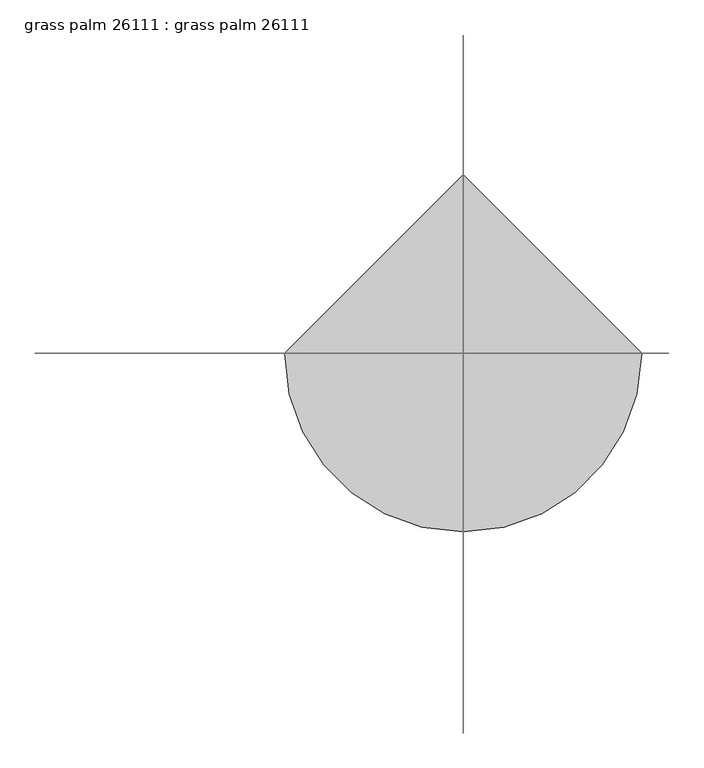
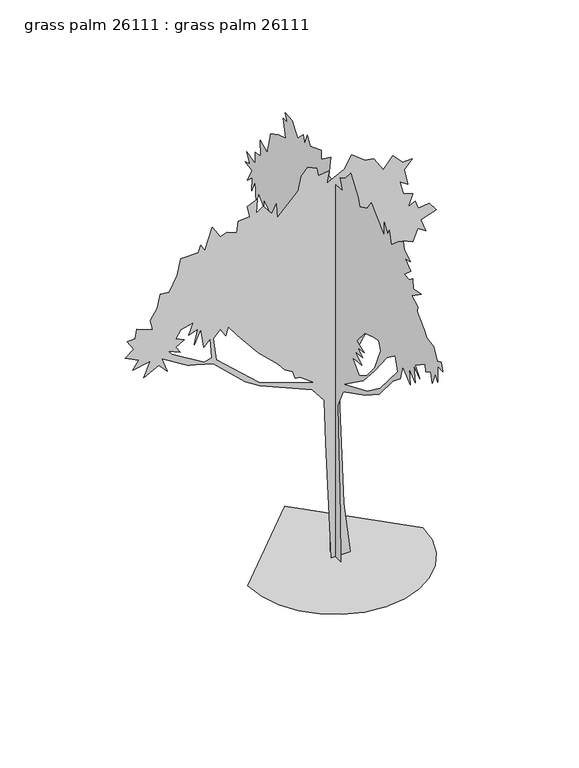
"""IFC4 building model written with IfcOpenShell, lengths in millimetres: proxy geometry, grass palm 26111 : grass palm 26111."""

from ifc_helpers import new_model, si_unit, origin, place, context, project, spatial, triangles, source, transform, mapped, element, save


def grass_palm_26111_grass_palm_26111_ffc4a38a(model_context):
    return source(origin(), model_context, "Body", "Tessellation", [
        triangles([(197.8251161, -0.0004657, 0.0001367), (109.1148514, -0.0002635, 694.5605118), (43.5490633, 0.0002048, 2380.5060047), (409.1686295, 0.0003079, 2962.5546341), (570.4154732, 0.000405, 3409.2137077), (607.6747178, 0.0004576, 3623.4372597), (719.4525244, 0.0004509, 3660.6992294), (654.2481468, 0.0004936, 3781.8063721), (747.397621, 0.0005252, 3949.4717194), (775.3401741, 0.0005007, 3874.9480705), (877.80376, 0.0005308, 4042.6134178), (1008.2098989, 0.0004934, 3977.4115837), (1073.4142765, 0.0005291, 4145.0772217), (1175.8753189, 0.0004934, 4070.5535728), (1110.6734848, 0.0005514, 4247.5407349), (1315.5981857, 0.0005381, 4312.742569), (1222.4487843, 0.0005851, 4433.8244225), (1082.7284609, 0.0006012, 4415.2060822), (1039.2334414, 0.0006388, 4529.6586891), (952.3222492, 0.0006386, 4480.4079163), (1008.2098989, 0.0006732, 4638.7514488), (886.9528381, 0.0007051, 4688.7640938), (840.544479, 0.0007593, 4862.3223953), (943.0055214, 0.0007261, 4797.0952721), (896.4321287, 0.0007914, 5011.3441132), (998.8957146, 0.0008063, 5123.1297318), (877.80376, 0.0008246, 5123.1297318), (747.397621, 0.0008797, 5253.5334), (626.3056664, 0.0008575, 5104.4861023), (503.8725509, 0.0009294, 5301.1072403), (384.1216845, 0.0009523, 5318.7352341), (216.4545022, 0.0010156, 5458.4604263), (113.9921609, 0.0009855, 5290.795079), (-109.5623986, 0.0009889, 5179.0094604), (-81.6183375, 0.0010277, 5337.3532837), (-221.3396873, 0.0010437, 5318.7352341), (-239.9693097, 0.0010769, 5430.5202713), (-361.0610281, 0.0011104, 5486.4005814), (-444.8937381, 0.0010978, 5393.2585922), (-482.1529827, 0.0010527, 5206.9496155), (-752.2819885, 0.0010175, 4927.5242294), (-770.9103573, 0.0010735, 5123.1297318), (-826.8005505, 0.0010516, 5011.3441132), (-938.5783207, 0.0011065, 5151.0698868), (-1031.7252514, 0.0011028, 5085.8680527), (-1013.0943392, 0.0011506, 5272.1514496), (-1143.5030216, 0.0011551, 5216.2711395), (-1115.557925, 0.0011104, 5067.2244232), (-1264.5950489, 0.0011304, 5057.9278976), (-1283.2232723, 0.0010926, 4908.8806), (-1404.3152996, 0.0011236, 4955.4643845), (-1497.4622303, 0.0011301, 4927.5242294), (-1599.9257435, 0.0011911, 5095.1895767), (-1702.389402, 0.0011281, 4806.4170868), (-1748.9628674, 0.0011604, 4899.5590759), (-1786.2220757, 0.0011407, 4806.4170868), (-2009.7751453, 0.0011745, 4806.4170868), (-2056.3486107, 0.0011233, 4592.1932442), (-2158.8122692, 0.0010856, 4396.5624527), (-2279.9041512, 0.0011064, 4405.8842674), (-2317.1635048, 0.0010639, 4228.8971054), (-2410.3102901, 0.00104, 4089.1972023), (-2377.0008408, 0.0009991, 3957.4473953), (-2587.2949814, 0.0010515, 4033.2916031), (-2605.9133217, 0.0010214, 3912.2100403), (-2708.3768349, 0.0010343, 3902.8882256), (-2624.5569511, 0.0009862, 3772.4845573), (-2736.3166992, 0.0009803, 3688.6390938), (-2559.355117, 0.0009282, 3595.4973953), (-2633.853186, 0.0009091, 3483.7117767), (-2410.3102901, 0.000888, 3530.2955612), (-2494.1431091, 0.0008475, 3334.6900589), (-2298.535136, 0.0008458, 3437.1535721), (-2186.7573658, 0.000796, 3316.0464294), (-2261.2733116, 0.0008604, 3511.6772209), (-1928.0074619, 0.0007539, 3305.1500015), (-1586.5374619, 0.000677, 3211.8556961), (-1169.4034029, 0.0005069, 2817.7745178), (-980.3029541, 0.0004448, 2694.5084953), (-299.9587802, 0.0002625, 2401.7378483), (-143.374379, 0.000185, 2203.9150394), (-126.1084725, 2.08e-05, 1609.6107628), (-53.6737587, -0.0004278, 0.0001367), (-1497.4622303, 0.0008957, 3651.4027039), (-1422.9462845, 0.000854, 3539.6173759), (-1395.0011879, 0.0008802, 3651.4027039), (-1273.9091606, 0.0008189, 3493.0335915), (-1002.0681953, 0.0003602, 3156.4073364), (-744.7432772, 0.0005791, 2905.2014488), (-659.9860233, 0.000538, 2801.1377426), (-556.6715083, 0.0005054, 2738.5520279), (-519.4122637, 0.0004719, 2636.0885147), (-454.2079225, 0.0004596, 2626.7667), (-267.9141337, 0.0003934, 2487.0438332), (-995.0831566, 0.0005747, 2749.8295372), (-1549.5677708, 0.0007954, 3253.765638), (-1590.6116318, 0.0008844, 3558.2354256), (-2019.0918732, 0.0008854, 3520.9737465), (-2074.9794502, 0.0009166, 3604.8192101), (-1963.20168, 0.0009175, 3670.0207535), (-2074.9794502, 0.0009495, 3725.9007729), (-2009.7751453, 0.0009676, 3828.3645767), (-1851.4239098, 0.0009538, 3865.6262558), (-1907.3141029, 0.0009217, 3716.604538), (-1791.7262455, 0.0009145, 3754.1964294), (-1838.0305412, 0.0008682, 3558.4641907), (-1748.9628674, 0.0009054, 3744.5444023), (-1711.7036591, 0.0008288, 3483.7117767), (-1627.8708401, 0.000839, 3567.5572403), (-1608.65835, 0.0007633, 3299.7651558), (-1708.7927902, 0.0007706, 3271.2916031), (-2130.8671726, 0.0009048, 3530.2955612), (-2177.4431087, 0.000927, 3586.1755806), (0.0001009, -125.9822357, 0.0001592), (6.27e-05, -114.0061317, 632.7801258), (3.21e-05, -52.0852428, 2115.3046051), (1.35e-05, -175.1038104, 2373.6836014), (-6.14e-05, -671.5328476, 2630.4243256), (-0.0001496, -990.5162842, 2836.0117767), (-0.0001562, -1298.9586491, 3200.2479744), (-0.0001816, -1467.3098557, 3334.6900589), (-0.00019, -1523.1974327, 3539.6173759), (-0.0002153, -1690.8629253, 3390.5700783), (-0.0002111, -1662.9202995, 3595.4973953), (-0.0002322, -1802.6406956, 3483.7373566), (-0.0002266, -1765.3814873, 3707.2827232), (-0.0002477, -1905.101738, 3604.8192101), (-0.0002322, -1802.6406956, 3725.9007729), (-0.000266, -2026.196236, 3874.9480705), (-0.0002688, -2044.8246048, 3781.8063721), (-0.0002843, -2147.2882633, 3837.6863914), (-0.0002899, -2184.5450008, 3707.2827232), (-0.0002997, -2249.7493057, 3874.9480705), (-0.0003096, -2314.9536106, 3800.4244217), (-0.0003096, -2314.9536106, 4023.9697884), (-0.0003265, -2426.7289101, 4014.6735535), (-0.0003208, -2389.4721725, 4126.4335922), (-0.0003068, -2296.3227711, 4079.8753876), (-0.0002955, -2221.8042091, 4238.2189201), (-0.0002716, -2063.4555897, 4266.1590752), (-0.0002632, -2007.5653965, 4340.6824333), (-0.0002792, -1849.2141609, 4489.729731), (-0.0002806, -1858.5282726, 4564.2280907), (-0.0002609, -1728.1221336, 4638.7514488), (-0.0002933, -1942.3609463, 4787.7987465), (-0.0002652, -1756.0672302, 4750.5370674), (-0.0002638, -1746.7531185, 4880.9404449), (-0.0002525, -1672.2345566, 4825.0607162), (-0.0002356, -1560.4567863, 4834.3569511), (-0.0002567, -1700.177037, 4955.4643845), (-0.0002384, -1579.0876259, 5057.9278976), (-0.0002553, -1690.8629253, 5085.8680527), (-0.0002342, -1551.1425293, 5169.6879364), (-0.0002314, -1532.5116898, 5262.854924), (-0.0002145, -1420.7339195, 5197.6530899), (-0.0001906, -1262.3826839, 5057.9278976), (-0.0001836, -1215.8092186, 5225.5932449), (-0.000178, -1178.5499376, 5151.0698868), (-0.0002067, -1104.0339191, 5272.1514496), (-0.0001667, -1104.0339191, 5085.8680527), (-0.0001811, -934.8191025, 5242.9666031), (-0.0001617, -805.9598167, 5355.9969131), (-0.0001497, -726.4933737, 5236.9472031), (-0.0001237, -554.4617231, 5151.0698868), (-0.0001181, -517.2024785, 5253.5334), (-9.28e-05, -349.5370585, 5486.4005814), (-7.45e-05, -228.4440684, 5346.6748077), (-5.62e-05, -107.3520956, 5281.4729736), (-6.46e-05, -163.2409807, 5132.4512558), (-4.21e-05, -14.2045188, 5123.1297318), (-1.82e-05, 144.1465339, 5151.0698868), (-2.38e-05, 106.8877798, 5430.5202713), (7.1e-06, 311.8129804, 5281.4729736), (7.1e-06, 311.8129804, 5402.5551178), (4.51e-05, 563.311074, 5309.4131287), (5.49e-05, 628.5154152, 5421.1987473), (6.48e-05, 693.7172493, 5262.854924), (6.9e-05, 721.6623459, 5365.3184372), (8.73e-05, 842.7543005, 5244.2112946), (9.71e-05, 907.9586054, 5309.4131287), (0.000107, 973.1604395, 5411.8766418), (9.09e-05, 1131.5116751, 5421.1987473), (0.0001238, 1084.9382097, 5318.7352341), (0.0001369, 1171.5319067, 5326.1010635), (0.0001281, 1112.8833063, 5085.8680527), (0.0001548, 1289.862838, 5020.6662186), (0.0001793, 1452.3822784, 4938.471817), (0.0001914, 1532.0468925, 4629.4296341), (0.0002153, 1690.3981281, 4703.9532829), (0.0002139, 1681.0838711, 4489.729731), (0.0002321, 1802.1758984, 4471.0861015), (0.0002321, 1802.1758984, 4312.742569), (0.0002617, 1997.7863422, 4359.3007736), (0.0002506, 1924.1873463, 4240.2763527), (0.0002671, 2033.8797787, 4204.1576271), (0.0002434, 1876.6944603, 4173.017086), (0.0002603, 1988.4722305, 3977.4115837), (0.000242, 1867.3802032, 4079.8753876), (0.0002448, 1886.008572, 3893.5664108), (0.0002321, 1802.1758984, 4070.5535728), (0.0002293, 1783.5475296, 3791.102607), (0.0002209, 1727.6573364, 3949.4717194), (0.000204, 1615.8795662, 3837.6863914), (0.000204, 1615.8795662, 3940.1499046), (0.0001974, 1307.620039, 3736.3911209), (0.0001385, 917.2727898, 3623.4372597), (0.0001194, 790.5928768, 3229.1531868), (0.0001184, 784.0523603, 3133.6235527), (0.0001019, 675.0888805, 3064.5609077), (0.0001273, 842.7543005, 2934.1575302), (0.0001104, 730.9765303, 2971.4192093), (0.0001532, 749.6048264, 2775.813707), (0.0001377, 647.143784, 2906.2173752), (0.0001349, 628.5154152, 2673.3501938), (0.0001307, 600.5703549, 2775.813707), (0.0001264, 572.6252584, 2673.3501938), (0.0001194, 526.0518293, 2841.0155411), (0.0001152, 498.1067327, 2682.6467194), (0.0001124, 479.478364, 2608.1483597), (0.0001067, 442.2191194, 2738.5520279), (9.69e-05, 377.0147781, 2654.7065643), (7.78e-05, 250.6550855, 2492.941729), (2.45e-05, 161.9890223, 2108.946999), (9.68e-05, 111.8545007, 1061.9156324), (0.0001375, 116.2017099, 0.0001159), (-9.51e-05, -630.0470804, 2801.0107155), (-0.0001338, -885.9978092, 3096.8699821), (-0.0001753, -1160.7521868, 3441.0905411), (-0.0002047, -1355.5320854, 3586.1755806), (-0.0002131, -1411.4196625, 3399.891893), (-0.0001538, -1018.750898, 2931.8969124), (-0.0001089, -721.0450871, 2712.8219124), (-2.89e-05, -191.1855686, 2487.0438332), (-6.83e-05, -451.9981009, 2980.7157349), (-8.93e-05, -591.7210041, 2990.0375496), (-6.83e-05, -451.9981009, 3092.5010628), (-9.36e-05, -619.6661007, 3111.1446922), (-7.67e-05, -507.7485861, 3183.8393829), (-9.92e-05, -656.9227655, 3204.2863907), (-7.39e-05, -489.2573819, 3269.4882248), (-0.0001003, -664.5148893, 3478.2763527), (-0.0001315, -871.1641943, 3548.9391907), (-0.0001484, -982.9419645, 3567.5572403), (-0.0001546, -1023.6937649, 3456.6608116), (-0.0001342, -889.0838854, 3136.1382248), (-0.0001091, -722.497978, 2934.7415062), (-8.09e-05, -535.8308109, 2813.0500969), (-5.98e-05, -396.1104876, 2971.4192093), (-1140.1273556, 0.0, 0.0001367), (-1109.9876982, -261.2415577, 0.0001834), (-1024.1458448, -501.1521864, 0.0002263), (-889.4750679, -712.8535812, 0.0002641), (-712.8535812, -889.4750679, 0.0002957), (-501.1496429, -1024.1458448, 0.0), (-261.2415577, -1109.9876982, 1.53e-05), (6.77e-05, -1140.1273556, 2.07e-05), (261.2415577, -1109.9876982, 1.53e-05), (501.1521864, -1024.1458448, 0.0), (712.8535812, -889.4750679, 0.0002957), (889.4750679, -712.8535812, 0.0002641), (1024.1458448, -501.1496429, 0.0002263), (1109.9876982, -261.2415577, 0.0001834), (1140.1273556, 9.97e-05, 0.0001367), (-0.0001476, 1140.1273556, 0.0002526)], [[95, 110, 96], [86, 3, 87], [87, 3, 88], [88, 3, 89], [106, 105, 107], [89, 3, 90], [90, 3, 91], [74, 73, 75], [42, 41, 43], [14, 13, 15], [98, 113, 99], [72, 71, 73], [96, 110, 97], [110, 109, 97], [70, 69, 71], [24, 23, 25], [26, 25, 27], [85, 84, 86], [55, 54, 56], [53, 52, 54], [104, 103, 105], [10, 9, 11], [108, 107, 109], [100, 99, 101], [46, 45, 47], [47, 45, 48], [66, 65, 67], [68, 67, 69], [16, 15, 17], [17, 15, 18], [35, 34, 36], [73, 71, 75], [64, 63, 65], [7, 6, 8], [3, 86, 4], [19, 18, 20], [32, 31, 33], [1, 83, 2], [83, 82, 2], [2, 82, 3], [82, 81, 3], [28, 27, 29], [12, 11, 13], [81, 80, 3], [4, 86, 5], [5, 86, 6], [21, 20, 22], [44, 43, 45], [27, 25, 29], [25, 23, 29], [60, 59, 61], [99, 113, 101], [49, 48, 50], [57, 56, 58], [6, 86, 8], [38, 37, 39], [37, 36, 39], [39, 36, 40], [36, 34, 40], [65, 63, 67], [67, 63, 69], [69, 63, 71], [71, 63, 75], [92, 91, 93], [91, 3, 93], [93, 3, 94], [3, 80, 94], [80, 79, 94], [94, 79, 95], [79, 78, 95], [95, 78, 110], [78, 77, 110], [110, 77, 111], [77, 76, 111], [111, 76, 112], [76, 75, 112], [112, 75, 113], [75, 63, 113], [113, 63, 101], [101, 63, 102], [97, 109, 84], [109, 107, 84], [8, 86, 9], [63, 62, 102], [62, 61, 102], [61, 59, 102], [102, 59, 103], [59, 58, 103], [58, 56, 103], [56, 54, 103], [18, 15, 20], [15, 13, 20], [13, 11, 20], [54, 52, 103], [52, 51, 103], [51, 50, 103], [103, 50, 105], [105, 50, 107], [107, 50, 84], [84, 50, 86], [86, 50, 9], [50, 48, 9], [48, 45, 9], [40, 34, 41], [30, 29, 31], [31, 29, 33], [33, 29, 34], [11, 9, 20], [29, 23, 34], [23, 22, 34], [34, 22, 41], [22, 20, 41], [20, 9, 41], [9, 45, 41], [45, 43, 41], [226, 245, 246], [245, 226, 227], [233, 116, 117], [126, 127, 128], [209, 210, 211], [198, 199, 200], [213, 214, 215], [196, 197, 198], [226, 246, 247], [200, 201, 202], [144, 145, 146], [238, 239, 240], [194, 195, 196], [218, 219, 220], [215, 216, 217], [158, 159, 160], [211, 212, 213], [245, 227, 228], [244, 245, 228], [131, 132, 133], [236, 237, 238], [234, 235, 236], [122, 123, 124], [133, 134, 135], [124, 125, 126], [156, 157, 158], [233, 226, 247], [192, 193, 194], [202, 203, 204], [151, 152, 153], [171, 172, 173], [175, 176, 177], [233, 117, 118], [232, 233, 118], [232, 118, 119], [231, 232, 119], [231, 119, 120], [230, 231, 120], [230, 120, 121], [217, 218, 220], [230, 121, 122], [229, 230, 122], [146, 147, 148], [177, 178, 179], [181, 182, 183], [188, 189, 190], [135, 136, 137], [135, 137, 138], [213, 215, 217], [173, 174, 175], [153, 154, 155], [183, 184, 185], [129, 130, 131], [165, 166, 167], [149, 150, 151], [161, 162, 163], [180, 181, 183], [192, 194, 196], [225, 114, 115], [224, 225, 115], [224, 115, 116], [223, 224, 116], [156, 158, 160], [233, 247, 248], [180, 183, 185], [179, 180, 185], [209, 211, 213], [167, 168, 169], [165, 167, 169], [164, 165, 169], [190, 191, 192], [248, 234, 236], [222, 223, 116], [222, 116, 233], [196, 198, 200], [222, 233, 248], [221, 222, 248], [220, 221, 248], [142, 143, 144], [217, 220, 248], [192, 196, 200], [151, 153, 155], [151, 155, 156], [149, 151, 156], [243, 244, 228], [243, 228, 229], [144, 146, 148], [144, 148, 149], [217, 248, 236], [138, 139, 140], [207, 208, 209], [200, 202, 204], [192, 200, 204], [190, 192, 204], [188, 190, 204], [188, 204, 205], [188, 205, 206], [209, 213, 217], [209, 217, 236], [209, 236, 238], [209, 238, 240], [207, 209, 240], [206, 207, 240], [206, 240, 241], [188, 206, 241], [187, 188, 241], [186, 187, 241], [185, 186, 241], [179, 185, 241], [177, 179, 241], [175, 177, 241], [173, 175, 241], [171, 173, 241], [170, 171, 241], [169, 170, 241], [164, 169, 241], [164, 241, 242], [164, 242, 243], [163, 164, 243], [161, 163, 243], [160, 161, 243], [160, 243, 229], [156, 160, 229], [149, 156, 229], [144, 149, 229], [142, 144, 229], [141, 142, 229], [141, 229, 122], [141, 122, 124], [141, 124, 126], [141, 126, 128], [141, 128, 129], [140, 141, 129], [138, 140, 129], [138, 129, 131], [138, 131, 133], [138, 133, 135], [263, 264, 249], [262, 263, 249], [262, 249, 250], [261, 262, 250], [261, 250, 251], [261, 251, 252], [260, 261, 252], [259, 260, 252], [259, 252, 253], [259, 253, 254], [259, 254, 255], [259, 255, 256], [259, 256, 257], [259, 257, 258]], closed=False),
    ])


if __name__ == "__main__":
    model = new_model("IFC4")
    model_context = context("Model", 3, world=origin())
    ifc_project = project(units=[si_unit("LENGTHUNIT", "METRE", prefix="MILLI")], contexts=[model_context])
    site = spatial("IfcSite", under=ifc_project)
    building = spatial("IfcBuilding", under=site)
    placement = place(None, origin())
    grass_palm_26111_grass_palm_26111_shape = grass_palm_26111_grass_palm_26111_ffc4a38a(model_context)
    element("IfcBuildingElementProxy", 1, Name="grass palm 26111 : grass palm 26111", ObjectType="grass palm 26111 : grass palm 26111", at=placement, inside=building, context=model_context, shape_type="MappedRepresentation", body=[
        mapped(grass_palm_26111_grass_palm_26111_shape, transform((0.0, 0.0, 0.0), x_axis=(1.0, 0.0, 0.0), y_axis=(0.0, 1.0, 0.0), z_axis=(0.0, 0.0, 1.0))),
    ])
    save(model, "model.ifc")

# Revit data of these elements
# Type "grass palm 26111 : grass palm 26111"
#   built-in parameter 1005195 = "RPC-16-FXGK-2WG0-PNFG-U000-ST1L-LVER-AU"
#   Height = 0
